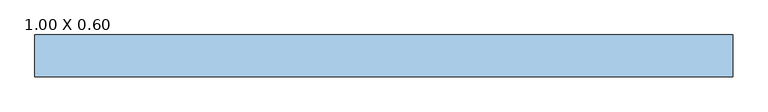
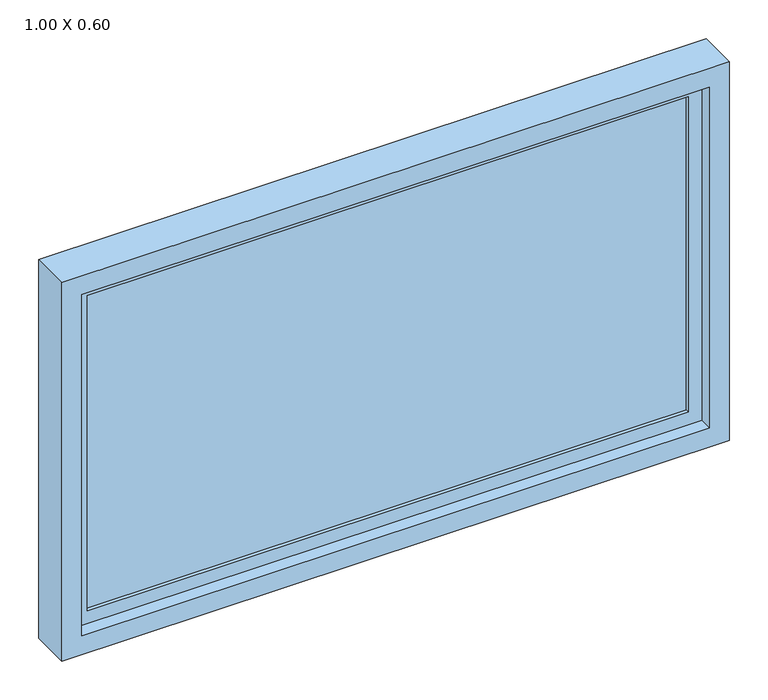
"""IFC4 building model written with IfcOpenShell, lengths in millimetres: window geometry, JANELA_MAXIM-AR_VIDRO : 1.00 X 0.60."""

from ifc_helpers import new_model, si_unit, frame, origin, place, context, project, spatial, polyline, outline, extrude, source, transform, mapped, element, save


def window_1_00_x_0_60_b119aca1(model_context):
    return source(origin(), model_context, "Body", "SweptSolid", [
        extrude(outline(polyline([(-450.0, 4.0), (450.0, 4.0), (450.0, -4.0), (-450.0, -4.0), (-450.0, 4.0)])), frame((0.0, 0.0, 1550.0), z_axis=(0.0, 0.0, 1.0), x_axis=(1.0, 0.0, 0.0)), (0.0, 0.0, 1.0), 500.0),
        extrude(outline(polyline([(1530.0, 470.0), (2070.0, 470.0), (2070.0, -470.0), (1530.0, -470.0), (1530.0, 470.0)]), holes=[polyline([(2050.0, 450.0), (1550.0, 450.0), (1550.0, -450.0), (2050.0, -450.0), (2050.0, 450.0)])]), frame((0.0, -10.0, 0.0), z_axis=(0.0, 1.0, 0.0), x_axis=(0.0, 0.0, 1.0)), (0.0, 0.0, 1.0), 20.0),
        extrude(outline(polyline([(2100.0, 500.0), (2100.0, -500.0), (1500.0, -500.0), (1500.0, 500.0), (2100.0, 500.0)]), holes=[polyline([(1530.0, 470.0), (1530.0, -470.0), (2070.0, -470.0), (2070.0, 470.0), (1530.0, 470.0)])]), frame((0.0, -30.0, 0.0), z_axis=(0.0, 1.0, 0.0), x_axis=(0.0, 0.0, 1.0)), (0.0, 0.0, 1.0), 60.0),
    ])


if __name__ == "__main__":
    model = new_model("IFC4")
    model_context = context("Model", 3, world=origin())
    ifc_project = project(units=[si_unit("LENGTHUNIT", "METRE", prefix="MILLI")], contexts=[model_context])
    site = spatial("IfcSite", under=ifc_project)
    building = spatial("IfcBuilding", under=site)
    placement = place(None, origin())
    window_1_00_x_0_60_shape = window_1_00_x_0_60_b119aca1(model_context)
    element("IfcWindow", 1, ObjectType="JANELA_MAXIM-AR_VIDRO : 1.00 X 0.60", at=placement, inside=building, context=model_context, shape_type="MappedRepresentation", body=[
        mapped(window_1_00_x_0_60_shape, transform((0.0, 0.0, 0.0), x_axis=(1.0, 0.0, 0.0), y_axis=(0.0, 1.0, 0.0), z_axis=(0.0, 0.0, 1.0))),
    ])
    save(model, "model.ifc")

# Revit data of these elements
# Type "JANELA_MAXIM-AR_VIDRO : 1.00 X 0.60"
#   Description = "Janela Maxim-Ar"
#   Type Mark = "J3"
#   Largura Painel [instance default] = 0.02 m
#   Largura Esquadria [instance default] = 0.06 m
#   Espessura Vidro [instance default] = 0.008 m
#   Espessura Painel [instance default] = 0.02 m
#   Espessura Esquadria [instance default] = 0.03 m
#   Height = 0.60 m
#   Altura-padrão do peitoril = 1.50 m
#   Width = 1.00 m
#   Vidro = .VIDRO
#   Esquadria = .ALUMÍNIO COM PINTURA ELETROSTÁTICA BRANCA
#   Wall Closure = (empty or 0)
# Element 1 (IfcWindow, "JANELA_MAXIM-AR_VIDRO : 1.00 X 0.60")
#   Materials on its faces: ".ALUMÍNIO COM PINTURA ELETROSTÁTICA BRANCA", ".VIDRO"
# Materials
#   ".VIDRO": class "Genérico", colour RGB 198 236 255, transparency 0.95, Cost = 0
#   ".ALUMÍNIO COM PINTURA ELETROSTÁTICA BRANCA": class "CC_METAIS", colour RGB 241 241 241, transparency 0, Cost = 0
